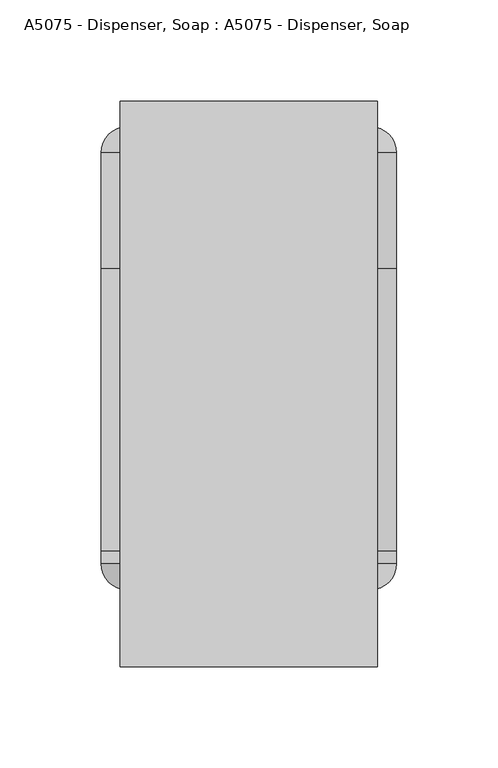
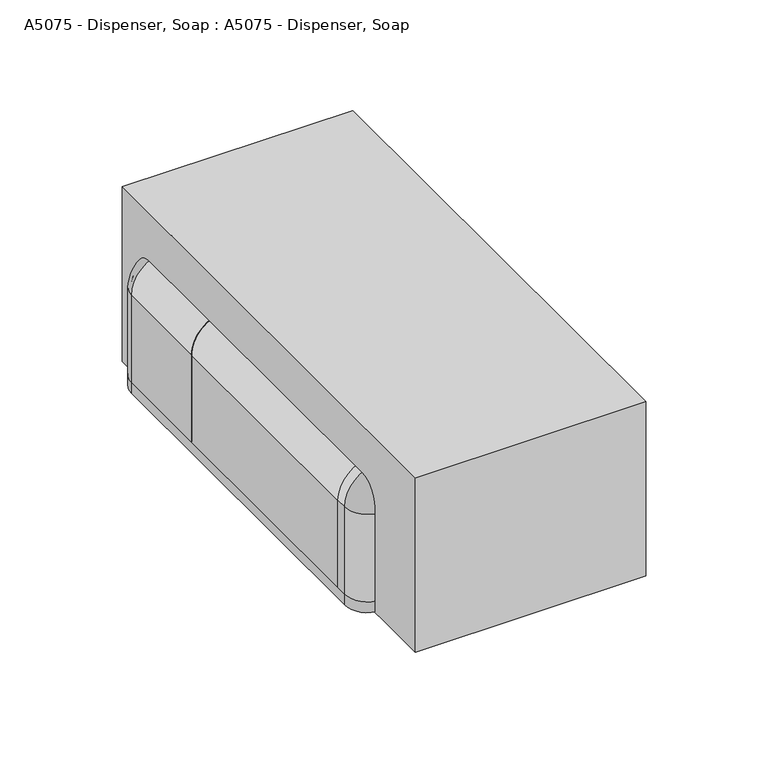
"""IFC4 building model written with IfcOpenShell, lengths in millimetres: proxy geometry, A5075 - Dispenser, Soap : A5075 - Dispenser, Soap."""

import ifcopenshell
import ifcopenshell.guid

model = None  # the IFC model being written
_history = None  # IfcOwnerHistory: only IFC2X3 demands one
_inside = {}  # id of a spatial element -> (the spatial element, [elements in it])
_under = {}  # id of a project, library or spatial element -> (it, [spatial elements below it])
_declared = {}  # id of a project -> (the project, [libraries it declares])
_typed = {}  # id of a type object -> (the type object, [elements of that type])
_made_of = {}  # id of a material, layer set ... -> (it, [elements and type objects made of it])


def new_model(schema):
    """Start an empty IFC model of exactly this schema.

    Asked for "IFC4X3", IfcOpenShell would pick the latest addendum, in which some entities
    have other attributes; the version numbers below select the first issue.
    IFC2X3 requires an IfcOwnerHistory on every rooted entity: one is made here for all.
    """
    global model, _history
    if schema == "IFC4X3":
        model = ifcopenshell.file(schema_version=(4, 3, 0, 0))
    else:
        model = ifcopenshell.file(schema=schema)
    _inside.clear()
    _under.clear()
    _declared.clear()
    _typed.clear()
    _made_of.clear()
    _history = None
    if model.schema == "IFC2X3":
        org = make("IfcOrganization", Name="unknown")
        user = make(
            "IfcPersonAndOrganization",
            ThePerson=make("IfcPerson", FamilyName="unknown"),
            TheOrganization=org,
        )
        app = make(
            "IfcApplication",
            ApplicationDeveloper=org,
            Version="unknown",
            ApplicationFullName="unknown",
            ApplicationIdentifier="unknown",
        )
        _history = make(
            "IfcOwnerHistory",
            OwningUser=user,
            OwningApplication=app,
            ChangeAction="ADDED",
            CreationDate=0,
        )
    return model


def make(cls, **values):
    """One entity of the class cls with the attributes given. An attribute that is None is left unset."""
    return model.create_entity(
        cls, **{name: value for name, value in values.items() if value is not None}
    )


def rooted(cls, **values):
    """An entity with a GlobalId (a new one), such as an element, a storey or a relation."""
    return make(cls, GlobalId=ifcopenshell.guid.new(), OwnerHistory=_history, **values)


def si_unit(unit_type, name, prefix=None):
    """IfcSIUnit, for example si_unit("LENGTHUNIT", "METRE", prefix="MILLI")."""
    return make("IfcSIUnit", UnitType=unit_type, Prefix=prefix, Name=name)


def assignment(units):
    """IfcUnitAssignment: the units of a project."""
    return None if units is None else make("IfcUnitAssignment", Units=units)


def point(xyz):
    """IfcCartesianPoint."""
    return None if xyz is None else make("IfcCartesianPoint", Coordinates=xyz)


def direction(xyz):
    """IfcDirection."""
    return None if xyz is None else make("IfcDirection", DirectionRatios=xyz)


def frame(location, z_axis=None, x_axis=None):
    """IfcAxis2Placement3D, a coordinate frame: its origin and axes. An axis left out is left unset."""
    return make(
        "IfcAxis2Placement3D",
        Location=point(location),
        Axis=direction(z_axis),
        RefDirection=direction(x_axis),
    )


def frame_2d(location, x_axis=None):
    """IfcAxis2Placement2D, a coordinate frame in the plane: its origin and x axis."""
    return make(
        "IfcAxis2Placement2D", Location=point(location), RefDirection=direction(x_axis)
    )


def origin():
    """The frame at (0, 0, 0) with its axes left unset."""
    return frame((0.0, 0.0, 0.0))


def origin_with_axes():
    """The frame at (0, 0, 0) with the z axis (0, 0, 1) and the x axis (1, 0, 0) written out."""
    return frame((0.0, 0.0, 0.0), z_axis=(0.0, 0.0, 1.0), x_axis=(1.0, 0.0, 0.0))


def place(relative_to, where):
    """IfcLocalPlacement: puts the frame where relative to a parent placement (None: the world)."""
    return make(
        "IfcLocalPlacement", PlacementRelTo=relative_to, RelativePlacement=where
    )


def context(
    kind, dimensions, precision=None, world=None, true_north=None, identifier=None
):
    """IfcGeometricRepresentationContext, for example the 3D "Model" context."""
    return make(
        "IfcGeometricRepresentationContext",
        ContextIdentifier=identifier,
        ContextType=kind,
        CoordinateSpaceDimension=dimensions,
        Precision=precision,
        WorldCoordinateSystem=world,
        TrueNorth=true_north,
    )


def project(units=None, contexts=None):
    """IfcProject with its units and contexts."""
    return rooted(
        "IfcProject",
        Name="project",
        RepresentationContexts=contexts,
        UnitsInContext=assignment(units),
    )


def spatial(cls, under=None, at=None, **own):
    """A site, building, storey or space (cls), placed at a placement, below another one or the project."""
    s = rooted(cls, ObjectPlacement=at, **own)
    if under is not None:
        _under.setdefault(under.id(), (under, []))[1].append(s)
    return s


def polyline(points):
    """IfcPolyline through the points."""
    return make("IfcPolyline", Points=[point(p) for p in points])


def circle_curve(where, radius):
    """IfcCircle in the frame where."""
    return make("IfcCircle", Position=where, Radius=radius)


def ellipse_curve(where, semi_axis1, semi_axis2):
    """IfcEllipse in the frame where."""
    return make(
        "IfcEllipse", Position=where, SemiAxis1=semi_axis1, SemiAxis2=semi_axis2
    )


def trimmed(basis, trim1, trim2, sense, master):
    """IfcTrimmedCurve: the piece of a basis curve between two trims."""
    return make(
        "IfcTrimmedCurve",
        BasisCurve=basis,
        Trim1=trim1,
        Trim2=trim2,
        SenseAgreement=sense,
        MasterRepresentation=master,
    )


def segment(curve, same_sense, transition):
    """IfcCompositeCurveSegment."""
    return make(
        "IfcCompositeCurveSegment",
        Transition=transition,
        SameSense=same_sense,
        ParentCurve=curve,
    )


def composite_curve(segments, self_intersect=None):
    """IfcCompositeCurve: segments joined end to end."""
    return make("IfcCompositeCurve", Segments=segments, SelfIntersect=self_intersect)


def outline(outer, holes=None, kind="AREA"):
    """IfcArbitraryClosedProfileDef: a profile drawn as a closed curve; with holes, ...WithVoids."""
    if holes is None:
        return make("IfcArbitraryClosedProfileDef", ProfileType=kind, OuterCurve=outer)
    return make(
        "IfcArbitraryProfileDefWithVoids",
        ProfileType=kind,
        OuterCurve=outer,
        InnerCurves=holes,
    )


def extrude(swept, where, along, depth):
    """IfcExtrudedAreaSolid: the profile swept, set in the frame where, extruded along a direction by depth."""
    return make(
        "IfcExtrudedAreaSolid",
        SweptArea=swept,
        Position=where,
        ExtrudedDirection=direction(along),
        Depth=depth,
    )


def shape(context_of_items, identifier, shape_type, items):
    """IfcShapeRepresentation: the items that make up one representation, for example the "Body"."""
    return make(
        "IfcShapeRepresentation",
        ContextOfItems=context_of_items,
        RepresentationIdentifier=identifier,
        RepresentationType=shape_type,
        Items=items,
    )


def source(mapping_origin, context_of_items, identifier, shape_type, items):
    """IfcRepresentationMap: a shape defined once, which mapped items show again and again."""
    return make(
        "IfcRepresentationMap",
        MappingOrigin=mapping_origin,
        MappedRepresentation=shape(context_of_items, identifier, shape_type, items),
    )


def transform(
    local_origin,
    x_axis=None,
    y_axis=None,
    z_axis=None,
    scale=None,
    scale2=None,
    scale3=None,
    uniform=True,
):
    """IfcCartesianTransformationOperator3D, or its non-uniform kind. x_axis, y_axis, z_axis: its Axis1, 2, 3."""
    if uniform:
        return make(
            "IfcCartesianTransformationOperator3D",
            Axis1=direction(x_axis),
            Axis2=direction(y_axis),
            LocalOrigin=point(local_origin),
            Scale=scale,
            Axis3=direction(z_axis),
        )
    return make(
        "IfcCartesianTransformationOperator3DnonUniform",
        Axis1=direction(x_axis),
        Axis2=direction(y_axis),
        LocalOrigin=point(local_origin),
        Scale=scale,
        Axis3=direction(z_axis),
        Scale2=scale2,
        Scale3=scale3,
    )


def mapped(mapping_source, mapping_target):
    """IfcMappedItem: shows the shape of a source again, moved by a transform."""
    return make(
        "IfcMappedItem", MappingSource=mapping_source, MappingTarget=mapping_target
    )


def made_of(thing, what):
    """Note that an element or type object is made of a material, layer set ...; save() writes the relation."""
    if what is not None:
        _made_of.setdefault(what.id(), (what, []))[1].append(thing)
    return thing


def element(
    cls,
    number,
    at=None,
    inside=None,
    cuts=None,
    type_object=None,
    material=None,
    context=None,
    identifier="Body",
    shape_type=None,
    held_by="IfcProductDefinitionShape",
    body=None,
    shapes=None,
    **own,
):
    """One element of the class cls, such as IfcWall. Its Tag is "e" and its number.

    at: its placement. inside: the storey or other place that contains it. cuts: it is an
    opening in that element (IfcRelVoidsElement). A single representation is given by context,
    identifier, shape_type and body (its items); several are given by shapes. held_by: the class
    of the entity that holds the representations. save() writes the other relations.
    """
    e = rooted(cls, Tag="e%d" % number, ObjectPlacement=at, **own)
    if body is not None:
        shapes = [shape(context, identifier, shape_type, body)]
    if shapes is not None:
        e.Representation = make(held_by, Representations=shapes)
    if inside is not None:
        _inside.setdefault(inside.id(), (inside, []))[1].append(e)
    if cuts is not None:
        rooted(
            "IfcRelVoidsElement", RelatingBuildingElement=cuts, RelatedOpeningElement=e
        )
    if type_object is not None:
        _typed.setdefault(type_object.id(), (type_object, []))[1].append(e)
    return made_of(e, material)


def aggregate(whole, parts):
    """IfcRelAggregates: a whole, such as a stair, and the parts it consists of."""
    return rooted("IfcRelAggregates", RelatingObject=whole, RelatedObjects=parts)


def save(model, path):
    """Write the relations noted so far, then the file.

    IfcRelAggregates (storeys below a building ...), IfcRelContainedInSpatialStructure (elements
    in a storey), IfcRelDefinesByType, IfcRelAssociatesMaterial and IfcRelDeclares: one each for
    every whole, place, type object, material and project.
    """
    for whole, parts in _under.values():
        aggregate(whole, parts)
    for where, things in _inside.values():
        rooted(
            "IfcRelContainedInSpatialStructure",
            RelatedElements=things,
            RelatingStructure=where,
        )
    for kind, things in _typed.values():
        rooted("IfcRelDefinesByType", RelatedObjects=things, RelatingType=kind)
    for what, things in _made_of.values():
        rooted("IfcRelAssociatesMaterial", RelatedObjects=things, RelatingMaterial=what)
    for by, libraries in _declared.values():
        rooted("IfcRelDeclares", RelatingContext=by, RelatedDefinitions=libraries)
    model.write(path)


def plane_surface(at):
    """IfcPlane: the flat surface through the origin of the frame at, square to its z axis."""
    return make("IfcPlane", Position=at)


def cylinder_surface(at, radius):
    """IfcCylindricalSurface: all points at the distance radius from the z axis of the frame at."""
    return make("IfcCylindricalSurface", Position=at, Radius=radius)


def revolved_surface(curve, axis_point, axis_direction):
    """IfcSurfaceOfRevolution: the curve turned about the line through axis_point along axis_direction."""
    return make(
        "IfcSurfaceOfRevolution",
        SweptCurve=make("IfcArbitraryOpenProfileDef", ProfileType="CURVE", Curve=curve),
        AxisPosition=make("IfcAxis1Placement", Location=point(axis_point), Axis=direction(axis_direction)),
    )


def advanced_brep(points, edges, surfaces, faces):
    """IfcAdvancedBrep: a solid bounded by faces that lie on surfaces and meet in shared edges.

    An edge is (start, end): straight between two places in points (the first is 0);
    or (start, end, curve); or (start, end, curve, False) where it runs against its curve.
    A face is (place in surfaces, loops), or (place, loops, False) where it looks against
    its surface's normal. A loop lists edges by number (the first is 1), with a minus sign
    where the edge is run from its end to its start. The first loop is the outer one.
    """
    corners = [point(p) for p in points]
    vertices = [make("IfcVertexPoint", VertexGeometry=c) for c in corners]
    made = []
    for start, end, *more in edges:
        made.append(
            make(
                "IfcEdgeCurve",
                EdgeStart=vertices[start],
                EdgeEnd=vertices[end],
                EdgeGeometry=more[0] if more else make("IfcPolyline", Points=[corners[start], corners[end]]),
                SameSense=more[1] if len(more) > 1 else True,
            )
        )
    hull = []
    for where, loops, *sense in faces:
        bounds = []
        for j, loop in enumerate(loops):
            ring = [make("IfcOrientedEdge", EdgeElement=made[abs(k) - 1], Orientation=k > 0) for k in loop]
            bounds.append(
                make(
                    "IfcFaceOuterBound" if j == 0 else "IfcFaceBound",
                    Bound=make("IfcEdgeLoop", EdgeList=ring),
                    Orientation=True,
                )
            )
        hull.append(make("IfcAdvancedFace", Bounds=bounds, FaceSurface=surfaces[where], SameSense=sense[0] if sense else True))
    return make("IfcAdvancedBrep", Outer=make("IfcClosedShell", CfsFaces=hull))


def a5075_dispenser_soap_a5075_dispenser_soap_cc7686cf(model_context):
    return source(origin(), model_context, "Body", "SolidModel", [
        advanced_brep(
        [(-73.025, -25.4, 6.35), (-60.325, -12.7, 6.35), (-60.325, -14.2875, 6.35), (-71.4375, -25.4, 6.35), (-71.4375, -82.55, 6.35), (-73.025, -82.55, 6.35), (-73.025, -82.55, 57.15), (-73.025, -25.4, 57.15), (-71.4375, -82.55, 57.15), (-53.975, -82.55, 74.6125), (53.975, -82.55, 74.6125), (71.4375, -82.55, 57.15), (71.4375, -82.55, 6.35), (73.025, -82.55, 6.35), (73.025, -82.55, 57.15), (53.975, -82.55, 76.2), (-53.975, -82.55, 76.2), (-71.4375, -25.4, 57.15), (-60.325, -14.2875, 57.15), (-60.325, -12.7, 57.15), (-53.975, -25.4, 76.2), (-53.975, -25.4, 74.6125), (-53.975, -14.2875, 63.5), (-53.975, -12.7, 63.5), (53.975, -25.4, 76.2), (53.975, -25.4, 74.6125), (53.975, -14.2875, 63.5), (53.975, -12.7, 63.5), (73.025, -25.4, 57.15), (71.4375, -25.4, 57.15), (60.325, -14.2875, 57.15), (60.325, -12.7, 57.15), (73.025, -25.4, 6.35), (71.4375, -25.4, 6.35), (60.325, -14.2875, 6.35), (60.325, -12.7, 6.35)],
        [
            (0, 1, circle_curve(frame((-60.325, -25.4, 6.35), z_axis=(0.0, 0.0, -1.0), x_axis=(1.0, 0.0, 0.0)), 12.7)),
            (1, 2),
            (2, 3, circle_curve(frame((-60.325, -25.4, 6.35), z_axis=(0.0, 0.0, 1.0), x_axis=(1.0, 0.0, 0.0)), 11.1125)),
            (3, 4),
            (4, 5),
            (5, 0),
            (5, 6),
            (6, 7),
            (7, 0),
            (4, 8),
            (8, 9, circle_curve(frame((-53.975, -82.55, 57.15), z_axis=(0.0, 1.0, 0.0), x_axis=(-1.0, 0.0, 0.0)), 17.4625)),
            (9, 10),
            (10, 11, circle_curve(frame((53.975, -82.55, 57.15), z_axis=(0.0, 1.0, 0.0), x_axis=(0.0, 0.0, 1.0)), 17.4625)),
            (11, 12),
            (12, 13),
            (13, 14),
            (14, 15, circle_curve(frame((53.975, -82.55, 57.15), z_axis=(0.0, -1.0, 0.0), x_axis=(0.0, 0.0, 1.0)), 19.05)),
            (15, 16),
            (16, 6, circle_curve(frame((-53.975, -82.55, 57.15), z_axis=(0.0, -1.0, 0.0), x_axis=(-1.0, 0.0, 0.0)), 19.05)),
            (3, 17),
            (17, 8),
            (2, 18),
            (18, 17, circle_curve(frame((-60.325, -25.4, 57.15), z_axis=(0.0, 0.0, 1.0), x_axis=(1.0, 0.0, 0.0)), 11.1125)),
            (1, 19),
            (19, 18),
            (7, 19, circle_curve(frame((-60.325, -25.4, 57.15), z_axis=(0.0, 0.0, -1.0), x_axis=(1.0, 0.0, 0.0)), 12.7)),
            (16, 20),
            (20, 7, circle_curve(frame((-53.975, -25.4, 57.15), z_axis=(0.0, -1.0, 0.0), x_axis=(-1.0, 0.0, 0.0)), 19.05)),
            (21, 9),
            (17, 21, circle_curve(frame((-53.975, -25.4, 57.15), z_axis=(0.0, 1.0, 0.0), x_axis=(-1.0, 0.0, 0.0)), 17.4625)),
            (22, 21, circle_curve(frame((-53.975, -25.4, 63.5), z_axis=(1.0, 0.0, 0.0), x_axis=(0.0, 0.0, -1.0)), 11.1125)),
            (18, 22, circle_curve(frame((-53.975, -14.2875, 57.15), z_axis=(0.0, 1.0, 0.0), x_axis=(-1.0, 0.0, 0.0)), 6.35)),
            (23, 22),
            (19, 23, circle_curve(frame((-53.975, -12.7, 57.15), z_axis=(0.0, 1.0, 0.0), x_axis=(-1.0, 0.0, 0.0)), 6.35)),
            (20, 23, circle_curve(frame((-53.975, -25.4, 63.5), z_axis=(-1.0, 0.0, 0.0), x_axis=(0.0, 0.0, -1.0)), 12.7)),
            (15, 24),
            (24, 20),
            (21, 25),
            (25, 10),
            (22, 26),
            (26, 25, circle_curve(frame((53.975, -25.4, 63.5), z_axis=(1.0, 0.0, 0.0), x_axis=(0.0, 0.0, -1.0)), 11.1125)),
            (23, 27),
            (27, 26),
            (24, 27, circle_curve(frame((53.975, -25.4, 63.5), z_axis=(-1.0, 0.0, 0.0), x_axis=(0.0, 0.0, -1.0)), 12.7)),
            (14, 28),
            (28, 24, circle_curve(frame((53.975, -25.4, 57.15), z_axis=(0.0, -1.0, 0.0), x_axis=(0.0, 0.0, 1.0)), 19.05)),
            (29, 11),
            (25, 29, circle_curve(frame((53.975, -25.4, 57.15), z_axis=(0.0, 1.0, 0.0), x_axis=(0.0, 0.0, 1.0)), 17.4625)),
            (30, 29, circle_curve(frame((60.325, -25.4, 57.15), z_axis=(0.0, 0.0, -1.0), x_axis=(-1.0, 0.0, 0.0)), 11.1125)),
            (26, 30, circle_curve(frame((53.975, -14.2875, 57.15), z_axis=(0.0, 1.0, 0.0), x_axis=(0.0, 0.0, 1.0)), 6.35)),
            (31, 30),
            (27, 31, circle_curve(frame((53.975, -12.7, 57.15), z_axis=(0.0, 1.0, 0.0), x_axis=(0.0, 0.0, 1.0)), 6.35)),
            (28, 31, circle_curve(frame((60.325, -25.4, 57.15), z_axis=(0.0, 0.0, 1.0), x_axis=(-1.0, 0.0, 0.0)), 12.7)),
            (32, 13),
            (12, 33),
            (33, 34, circle_curve(frame((60.325, -25.4, 6.35), z_axis=(0.0, 0.0, 1.0), x_axis=(-1.0, 0.0, 0.0)), 11.1125)),
            (34, 35),
            (35, 32, circle_curve(frame((60.325, -25.4, 6.35), z_axis=(0.0, 0.0, -1.0), x_axis=(-1.0, 0.0, 0.0)), 12.7)),
            (32, 28),
            (29, 33),
            (30, 34),
            (31, 35),
        ],
        [
            plane_surface(frame((-73.025, -12.7, 6.35), z_axis=(0.0, 0.0, -1.0), x_axis=(0.0, -1.0, 0.0))),
            plane_surface(frame((-73.025, -25.4, 6.35), z_axis=(-1.0, 0.0, 0.0), x_axis=(0.0, 0.0, 1.0))),
            plane_surface(frame((-73.025, -82.55, 6.35), z_axis=(0.0, -1.0, 0.0), x_axis=(0.0, 0.0, 1.0))),
            plane_surface(frame((-71.4375, -82.55, 6.35), z_axis=(1.0, 0.0, 0.0), x_axis=(0.0, 0.0, 1.0))),
            revolved_surface(polyline([(-49.212500000000006, -25.4, 57.15), (-49.212500000000006, -25.4, 6.35)]), (-60.325, -25.4, 6.35), (0.0, 0.0, 1.0)),
            plane_surface(frame((-60.325, -14.2875, 6.35), z_axis=(1.0, 0.0, 0.0), x_axis=(0.0, 0.0, 1.0))),
            cylinder_surface(frame((-60.325, -25.4, 6.35), z_axis=(0.0, 0.0, -1.0), x_axis=(1.0, 0.0, 0.0)), 12.7),
            cylinder_surface(frame((-53.975, -12.7, 57.15), z_axis=(0.0, -1.0, 0.0), x_axis=(-1.0, 0.0, 0.0)), 19.05),
            revolved_surface(polyline([(-71.4375, -82.55, 57.15), (-71.4375, -25.4, 57.15)]), (-53.975, -12.7, 57.15), (0.0, -1.0, 0.0)),
            revolved_surface(trimmed(ellipse_curve(frame((-60.325, -25.4, 57.15), z_axis=(0.0, 0.0, -1.0), x_axis=(1.0, 0.0, 0.0)), 11.1125, 11.1125), [point((-71.4375, -25.4, 57.15))], [point((-60.325, -14.2875, 57.15))], True, "CARTESIAN"), (-53.975, -12.7, 57.15), (0.0, -1.0, 0.0)),
            revolved_surface(polyline([(-60.325, -14.2875, 57.15), (-60.325, -12.7, 57.15)]), (-53.975, -12.7, 57.15), (0.0, -1.0, 0.0)),
            revolved_surface(trimmed(ellipse_curve(frame((-60.325, -25.4, 57.15), z_axis=(0.0, 0.0, 1.0), x_axis=(1.0, 0.0, 0.0)), 12.7, 12.7), [point((-60.325, -12.7, 57.15))], [point((-73.025, -25.4, 57.15))], True, "CARTESIAN"), (-53.975, -12.7, 57.15), (0.0, -1.0, 0.0)),
            plane_surface(frame((-53.975, -25.4, 76.2), z_axis=(0.0, 0.0, 1.0), x_axis=(1.0, 0.0, 0.0))),
            plane_surface(frame((-53.975, -82.55, 74.6125), z_axis=(0.0, 0.0, -1.0), x_axis=(1.0, 0.0, 0.0))),
            revolved_surface(polyline([(53.975, -25.4, 52.3875), (-53.975, -25.4, 52.3875)]), (-53.975, -25.4, 63.5), (1.0, 0.0, 0.0)),
            plane_surface(frame((-53.975, -14.2875, 63.5), z_axis=(0.0, 0.0, -1.0), x_axis=(1.0, 0.0, 0.0))),
            cylinder_surface(frame((-53.975, -25.4, 63.5), z_axis=(-1.0, 0.0, 0.0), x_axis=(0.0, 0.0, -1.0)), 12.7),
            cylinder_surface(frame((53.975, -12.7, 57.15), z_axis=(0.0, -1.0, 0.0), x_axis=(0.0, 0.0, 1.0)), 19.05),
            revolved_surface(polyline([(53.975, -82.55, 74.6125), (53.975, -25.4, 74.6125)]), (53.975, -12.7, 57.15), (0.0, -1.0, 0.0)),
            revolved_surface(trimmed(ellipse_curve(frame((53.975, -25.4, 63.5), z_axis=(-1.0, 0.0, 0.0), x_axis=(0.0, 0.0, -1.0)), 11.1125, 11.1125), [point((53.975, -25.4, 74.6125))], [point((53.975, -14.2875, 63.5))], True, "CARTESIAN"), (53.975, -12.7, 57.15), (0.0, -1.0, 0.0)),
            revolved_surface(polyline([(53.975, -14.2875, 63.5), (53.975, -12.7, 63.5)]), (53.975, -12.7, 57.15), (0.0, -1.0, 0.0)),
            revolved_surface(trimmed(ellipse_curve(frame((53.975, -25.4, 63.5), z_axis=(1.0, 0.0, 0.0), x_axis=(0.0, 0.0, -1.0)), 12.7, 12.7), [point((53.975, -12.7, 63.5))], [point((53.975, -25.4, 76.2))], True, "CARTESIAN"), (53.975, -12.7, 57.15), (0.0, -1.0, 0.0)),
            plane_surface(frame((73.025, -12.7, 6.35), z_axis=(0.0, 0.0, -1.0), x_axis=(0.0, -1.0, 0.0))),
            plane_surface(frame((73.025, -25.4, 57.15), z_axis=(1.0, 0.0, 0.0), x_axis=(0.0, 0.0, -1.0))),
            plane_surface(frame((71.4375, -82.55, 57.15), z_axis=(-1.0, 0.0, 0.0), x_axis=(0.0, 0.0, -1.0))),
            revolved_surface(polyline([(49.212500000000006, -25.4, 6.350000000000001), (49.212500000000006, -25.4, 57.15)]), (60.325, -25.4, 57.15), (0.0, 0.0, -1.0)),
            plane_surface(frame((60.325, -14.2875, 57.15), z_axis=(-1.0, 0.0, 0.0), x_axis=(0.0, 0.0, -1.0))),
            cylinder_surface(frame((60.325, -25.4, 57.15), z_axis=(0.0, 0.0, 1.0), x_axis=(-1.0, 0.0, 0.0)), 12.7),
        ],
        [
            (0, [[1, 2, 3, 4, 5, 6]]),
            (1, [[7, 8, 9, -6]]),
            (2, [[10, 11, 12, 13, 14, 15, 16, 17, 18, 19, -7, -5]]),
            (3, [[20, 21, -10, -4]]),
            (4, [[22, 23, -20, -3]]),
            (5, [[24, 25, -22, -2]]),
            (6, [[-9, 26, -24, -1]]),
            (7, [[27, 28, -8, -19]]),
            (8, [[29, -11, -21, 30]]),
            (9, [[31, -30, -23, 32]]),
            (10, [[33, -32, -25, 34]]),
            (11, [[35, -34, -26, -28]]),
            (12, [[-18, 36, 37, -27]]),
            (13, [[38, 39, -12, -29]]),
            (14, [[40, 41, -38, -31]]),
            (15, [[42, 43, -40, -33]]),
            (16, [[-37, 44, -42, -35]]),
            (17, [[45, 46, -36, -17]]),
            (18, [[47, -13, -39, 48]]),
            (19, [[49, -48, -41, 50]]),
            (20, [[51, -50, -43, 52]]),
            (21, [[53, -52, -44, -46]]),
            (22, [[54, -15, 55, 56, 57, 58]]),
            (23, [[-16, -54, 59, -45]]),
            (24, [[60, -55, -14, -47]]),
            (25, [[61, -56, -60, -49]]),
            (26, [[62, -57, -61, -51]]),
            (27, [[-59, -58, -62, -53]]),
        ],
    ),
        advanced_brep(
        [(-73.025, -228.6, 6.35), (-73.025, -222.25, 6.35), (-71.4375, -222.25, 6.35), (-71.4375, -228.6, 6.35), (-60.325, -239.7125, 6.35), (-60.325, -241.3, 6.35), (-60.325, -241.3, 57.15), (-73.025, -228.6, 57.15), (-60.325, -239.7125, 57.15), (-71.4375, -228.6, 57.15), (-71.4375, -222.25, 57.15), (-73.025, -222.25, 57.15), (-53.975, -222.25, 76.2), (53.975, -222.25, 76.2), (73.025, -222.25, 57.15), (73.025, -222.25, 6.35), (71.4375, -222.25, 6.35), (71.4375, -222.25, 57.15), (53.975, -222.25, 74.6125), (-53.975, -222.25, 74.6125), (-53.975, -241.3, 63.5), (-53.975, -228.6, 76.2), (-53.975, -239.7125, 63.5), (-53.975, -228.6, 74.6125), (53.975, -241.3, 63.5), (53.975, -228.6, 76.2), (53.975, -239.7125, 63.5), (53.975, -228.6, 74.6125), (60.325, -241.3, 57.15), (73.025, -228.6, 57.15), (60.325, -239.7125, 57.15), (71.4375, -228.6, 57.15), (73.025, -228.6, 6.35), (60.325, -241.3, 6.35), (60.325, -239.7125, 6.35), (71.4375, -228.6, 6.35)],
        [
            (0, 1),
            (1, 2),
            (2, 3),
            (3, 4, circle_curve(frame((-60.325, -228.6, 6.35), z_axis=(0.0, 0.0, 1.0), x_axis=(1.0, 0.0, 0.0)), 11.1125)),
            (4, 5),
            (5, 0, circle_curve(frame((-60.325, -228.6, 6.35), z_axis=(0.0, 0.0, -1.0), x_axis=(1.0, 0.0, 0.0)), 12.7)),
            (5, 6),
            (6, 7, circle_curve(frame((-60.325, -228.6, 57.15), z_axis=(0.0, 0.0, -1.0), x_axis=(1.0, 0.0, 0.0)), 12.7)),
            (7, 0),
            (4, 8),
            (8, 6),
            (3, 9),
            (9, 8, circle_curve(frame((-60.325, -228.6, 57.15), z_axis=(0.0, 0.0, 1.0), x_axis=(1.0, 0.0, 0.0)), 11.1125)),
            (2, 10),
            (10, 9),
            (1, 11),
            (11, 12, circle_curve(frame((-53.975, -222.25, 57.15), z_axis=(0.0, 1.0, 0.0), x_axis=(-1.0, 0.0, 0.0)), 19.05)),
            (12, 13),
            (13, 14, circle_curve(frame((53.975, -222.25, 57.15), z_axis=(0.0, 1.0, 0.0), x_axis=(0.0, 0.0, 1.0)), 19.05)),
            (14, 15),
            (15, 16),
            (16, 17),
            (17, 18, circle_curve(frame((53.975, -222.25, 57.15), z_axis=(0.0, -1.0, 0.0), x_axis=(0.0, 0.0, 1.0)), 17.4625)),
            (18, 19),
            (19, 10, circle_curve(frame((-53.975, -222.25, 57.15), z_axis=(0.0, -1.0, 0.0), x_axis=(-1.0, 0.0, 0.0)), 17.4625)),
            (7, 11),
            (20, 21, circle_curve(frame((-53.975, -228.6, 63.5), z_axis=(-1.0, 0.0, 0.0), x_axis=(0.0, 0.0, -1.0)), 12.7)),
            (21, 7, circle_curve(frame((-53.975, -228.6, 57.15), z_axis=(0.0, -1.0, 0.0), x_axis=(-1.0, 0.0, 0.0)), 19.05)),
            (6, 20, circle_curve(frame((-53.975, -241.3, 57.15), z_axis=(0.0, 1.0, 0.0), x_axis=(-1.0, 0.0, 0.0)), 6.35)),
            (22, 20),
            (8, 22, circle_curve(frame((-53.975, -239.7125, 57.15), z_axis=(0.0, 1.0, 0.0), x_axis=(-1.0, 0.0, 0.0)), 6.35)),
            (23, 22, circle_curve(frame((-53.975, -228.6, 63.5), z_axis=(1.0, 0.0, 0.0), x_axis=(0.0, 0.0, -1.0)), 11.1125)),
            (9, 23, circle_curve(frame((-53.975, -228.6, 57.15), z_axis=(0.0, 1.0, 0.0), x_axis=(-1.0, 0.0, 0.0)), 17.4625)),
            (19, 23),
            (21, 12),
            (20, 24),
            (24, 25, circle_curve(frame((53.975, -228.6, 63.5), z_axis=(-1.0, 0.0, 0.0), x_axis=(0.0, 0.0, -1.0)), 12.7)),
            (25, 21),
            (22, 26),
            (26, 24),
            (23, 27),
            (27, 26, circle_curve(frame((53.975, -228.6, 63.5), z_axis=(1.0, 0.0, 0.0), x_axis=(0.0, 0.0, -1.0)), 11.1125)),
            (18, 27),
            (25, 13),
            (28, 29, circle_curve(frame((60.325, -228.6, 57.15), z_axis=(0.0, 0.0, 1.0), x_axis=(-1.0, 0.0, 0.0)), 12.7)),
            (29, 25, circle_curve(frame((53.975, -228.6, 57.15), z_axis=(0.0, -1.0, 0.0), x_axis=(0.0, 0.0, 1.0)), 19.05)),
            (24, 28, circle_curve(frame((53.975, -241.3, 57.15), z_axis=(0.0, 1.0, 0.0), x_axis=(0.0, 0.0, 1.0)), 6.35)),
            (30, 28),
            (26, 30, circle_curve(frame((53.975, -239.7125, 57.15), z_axis=(0.0, 1.0, 0.0), x_axis=(0.0, 0.0, 1.0)), 6.35)),
            (31, 30, circle_curve(frame((60.325, -228.6, 57.15), z_axis=(0.0, 0.0, -1.0), x_axis=(-1.0, 0.0, 0.0)), 11.1125)),
            (27, 31, circle_curve(frame((53.975, -228.6, 57.15), z_axis=(0.0, 1.0, 0.0), x_axis=(0.0, 0.0, 1.0)), 17.4625)),
            (17, 31),
            (29, 14),
            (32, 33, circle_curve(frame((60.325, -228.6, 6.35), z_axis=(0.0, 0.0, -1.0), x_axis=(-1.0, 0.0, 0.0)), 12.7)),
            (33, 34),
            (34, 35, circle_curve(frame((60.325, -228.6, 6.35), z_axis=(0.0, 0.0, 1.0), x_axis=(-1.0, 0.0, 0.0)), 11.1125)),
            (35, 16),
            (15, 32),
            (28, 33),
            (32, 29),
            (30, 34),
            (31, 35),
        ],
        [
            plane_surface(frame((-73.025, -241.3, 6.35), z_axis=(0.0, 0.0, -1.0), x_axis=(0.0, -1.0, 0.0))),
            cylinder_surface(frame((-60.325, -228.6, 6.35), z_axis=(0.0, 0.0, -1.0), x_axis=(1.0, 0.0, 0.0)), 12.7),
            plane_surface(frame((-60.325, -241.3, 6.35), z_axis=(1.0, 0.0, 0.0), x_axis=(0.0, 0.0, 1.0))),
            revolved_surface(polyline([(-49.212500000000006, -228.6, 57.15), (-49.212500000000006, -228.6, 6.35)]), (-60.325, -228.6, 6.35), (0.0, 0.0, 1.0)),
            plane_surface(frame((-71.4375, -228.6, 6.35), z_axis=(1.0, 0.0, 0.0), x_axis=(0.0, 0.0, 1.0))),
            plane_surface(frame((-71.4375, -222.25, 6.35), z_axis=(0.0, 1.0, 0.0), x_axis=(0.0, 0.0, 1.0))),
            plane_surface(frame((-73.025, -222.25, 6.35), z_axis=(-1.0, 0.0, 0.0), x_axis=(0.0, 0.0, 1.0))),
            revolved_surface(trimmed(ellipse_curve(frame((-60.325, -228.6, 57.15), z_axis=(0.0, 0.0, 1.0), x_axis=(1.0, 0.0, 0.0)), 12.7, 12.7), [point((-73.025, -228.6, 57.15))], [point((-60.325, -241.3, 57.15))], True, "CARTESIAN"), (-53.975, -241.3, 57.15), (0.0, -1.0, 0.0)),
            revolved_surface(polyline([(-60.325, -241.3, 57.15), (-60.325, -239.7125, 57.15)]), (-53.975, -241.3, 57.15), (0.0, -1.0, 0.0)),
            revolved_surface(trimmed(ellipse_curve(frame((-60.325, -228.6, 57.15), z_axis=(0.0, 0.0, -1.0), x_axis=(1.0, 0.0, 0.0)), 11.1125, 11.1125), [point((-60.325, -239.7125, 57.15))], [point((-71.4375, -228.6, 57.15))], True, "CARTESIAN"), (-53.975, -241.3, 57.15), (0.0, -1.0, 0.0)),
            revolved_surface(polyline([(-71.4375, -228.6, 57.15), (-71.4375, -222.25, 57.15)]), (-53.975, -241.3, 57.15), (0.0, -1.0, 0.0)),
            cylinder_surface(frame((-53.975, -241.3, 57.15), z_axis=(0.0, -1.0, 0.0), x_axis=(-1.0, 0.0, 0.0)), 19.05),
            cylinder_surface(frame((-53.975, -228.6, 63.5), z_axis=(-1.0, 0.0, 0.0), x_axis=(0.0, 0.0, -1.0)), 12.7),
            plane_surface(frame((-53.975, -241.3, 63.5), z_axis=(0.0, 0.0, -1.0), x_axis=(1.0, 0.0, 0.0))),
            revolved_surface(polyline([(53.975, -228.6, 52.3875), (-53.975, -228.6, 52.3875)]), (-53.975, -228.6, 63.5), (1.0, 0.0, 0.0)),
            plane_surface(frame((-53.975, -228.6, 74.6125), z_axis=(0.0, 0.0, -1.0), x_axis=(1.0, 0.0, 0.0))),
            plane_surface(frame((-53.975, -222.25, 76.2), z_axis=(0.0, 0.0, 1.0), x_axis=(1.0, 0.0, 0.0))),
            revolved_surface(trimmed(ellipse_curve(frame((53.975, -228.6, 63.5), z_axis=(1.0, 0.0, 0.0), x_axis=(0.0, 0.0, -1.0)), 12.7, 12.7), [point((53.975, -228.6, 76.2))], [point((53.975, -241.3, 63.5))], True, "CARTESIAN"), (53.975, -241.3, 57.15), (0.0, -1.0, 0.0)),
            revolved_surface(polyline([(53.975, -241.3, 63.5), (53.975, -239.7125, 63.5)]), (53.975, -241.3, 57.15), (0.0, -1.0, 0.0)),
            revolved_surface(trimmed(ellipse_curve(frame((53.975, -228.6, 63.5), z_axis=(-1.0, 0.0, 0.0), x_axis=(0.0, 0.0, -1.0)), 11.1125, 11.1125), [point((53.975, -239.7125, 63.5))], [point((53.975, -228.6, 74.6125))], True, "CARTESIAN"), (53.975, -241.3, 57.15), (0.0, -1.0, 0.0)),
            revolved_surface(polyline([(53.975, -228.6, 74.6125), (53.975, -222.25, 74.6125)]), (53.975, -241.3, 57.15), (0.0, -1.0, 0.0)),
            cylinder_surface(frame((53.975, -241.3, 57.15), z_axis=(0.0, -1.0, 0.0), x_axis=(0.0, 0.0, 1.0)), 19.05),
            plane_surface(frame((73.025, -241.3, 6.35), z_axis=(0.0, 0.0, -1.0), x_axis=(0.0, -1.0, 0.0))),
            cylinder_surface(frame((60.325, -228.6, 57.15), z_axis=(0.0, 0.0, 1.0), x_axis=(-1.0, 0.0, 0.0)), 12.7),
            plane_surface(frame((60.325, -241.3, 57.15), z_axis=(-1.0, 0.0, 0.0), x_axis=(0.0, 0.0, -1.0))),
            revolved_surface(polyline([(49.212500000000006, -228.6, 6.350000000000001), (49.212500000000006, -228.6, 57.15)]), (60.325, -228.6, 57.15), (0.0, 0.0, -1.0)),
            plane_surface(frame((71.4375, -228.6, 57.15), z_axis=(-1.0, 0.0, 0.0), x_axis=(0.0, 0.0, -1.0))),
            plane_surface(frame((73.025, -222.25, 57.15), z_axis=(1.0, 0.0, 0.0), x_axis=(0.0, 0.0, -1.0))),
        ],
        [
            (0, [[1, 2, 3, 4, 5, 6]]),
            (1, [[7, 8, 9, -6]]),
            (2, [[10, 11, -7, -5]]),
            (3, [[12, 13, -10, -4]]),
            (4, [[14, 15, -12, -3]]),
            (5, [[16, 17, 18, 19, 20, 21, 22, 23, 24, 25, -14, -2]]),
            (6, [[-9, 26, -16, -1]]),
            (7, [[27, 28, -8, 29]]),
            (8, [[30, -29, -11, 31]]),
            (9, [[32, -31, -13, 33]]),
            (10, [[34, -33, -15, -25]]),
            (11, [[35, -17, -26, -28]]),
            (12, [[36, 37, 38, -27]]),
            (13, [[39, 40, -36, -30]]),
            (14, [[41, 42, -39, -32]]),
            (15, [[-24, 43, -41, -34]]),
            (16, [[-38, 44, -18, -35]]),
            (17, [[45, 46, -37, 47]]),
            (18, [[48, -47, -40, 49]]),
            (19, [[50, -49, -42, 51]]),
            (20, [[52, -51, -43, -23]]),
            (21, [[53, -19, -44, -46]]),
            (22, [[54, 55, 56, 57, -21, 58]]),
            (23, [[59, -54, 60, -45]]),
            (24, [[61, -55, -59, -48]]),
            (25, [[62, -56, -61, -50]]),
            (26, [[-22, -57, -62, -52]]),
            (27, [[-60, -58, -20, -53]]),
        ],
    ),
        extrude(outline(composite_curve([segment(polyline([(57.15, -73.025), (6.35, -73.025), (6.35, -71.4375), (57.15, -71.4375)]), True, "CONTINUOUS"), segment(trimmed(circle_curve(frame_2d((57.15, -53.975)), 17.4625), [point((57.15, -71.4375))], [point((74.6125, -53.975))], True, "CARTESIAN"), True, "CONTINUOUS"), segment(polyline([(74.6125, -53.975), (74.6125, 53.975)]), True, "CONTINUOUS"), segment(trimmed(circle_curve(frame_2d((57.15, 53.975)), 17.4625), [point((74.6125, 53.975))], [point((57.15, 71.4375))], True, "CARTESIAN"), True, "CONTINUOUS"), segment(polyline([(57.15, 71.4375), (6.35, 71.4375), (6.35, 73.025), (57.15, 73.025)]), True, "CONTINUOUS"), segment(trimmed(circle_curve(frame_2d((57.15, 53.975)), 19.05), [point((57.15, 73.025))], [point((76.2, 53.975))], False, "CARTESIAN"), True, "CONTINUOUS"), segment(polyline([(76.2, 53.975), (76.2, -53.975)]), True, "CONTINUOUS"), segment(trimmed(circle_curve(frame_2d((57.15, -53.975)), 19.05), [point((76.2, -53.975))], [point((57.15, -73.025))], False, "CARTESIAN"), True, "CONTINUOUS")], self_intersect=False)), frame((0.0, -222.25, 0.0), z_axis=(0.0, 1.0, 0.0), x_axis=(0.0, 0.0, 1.0)), (0.0, 0.0, 1.0), 139.7),
        extrude(outline(composite_curve([segment(polyline([(74.6125, 53.975), (74.6125, -53.975)]), True, "CONTINUOUS"), segment(trimmed(circle_curve(frame_2d((57.15, -53.975)), 17.4625), [point((74.6125, -53.975))], [point((57.15, -71.4375))], False, "CARTESIAN"), True, "CONTINUOUS"), segment(polyline([(57.15, -71.4375), (6.35, -71.4375), (6.35, 71.4375), (57.15, 71.4375)]), True, "CONTINUOUS"), segment(trimmed(circle_curve(frame_2d((57.15, 53.975)), 17.4625), [point((57.15, 71.4375))], [point((74.6125, 53.975))], False, "CARTESIAN"), True, "CONTINUOUS")], self_intersect=False)), frame((0.0, -184.4030988, 0.0), z_axis=(0.0, 1.0, 0.0), x_axis=(0.0, 0.0, 1.0)), (0.0, 0.0, 1.0), 101.8530988),
        extrude(outline(composite_curve([segment(trimmed(circle_curve(frame_2d((47.625, 0.0)), 9.525), [point((47.625, -9.525))], [point((47.625, 9.525))], False, "CARTESIAN"), True, "CONTINUOUS"), segment(trimmed(circle_curve(frame_2d((47.625, 0.0)), 9.525), [point((47.625, 9.525))], [point((47.625, -9.525))], False, "CARTESIAN"), True, "CONTINUOUS")], self_intersect=False)), frame((0.0, -12.7, 0.0), z_axis=(0.0, 1.0, 0.0), x_axis=(0.0, 0.0, 1.0)), (0.0, 0.0, 1.0), 12.7),
        extrude(outline(composite_curve([segment(trimmed(circle_curve(frame_2d((-9.525, -41.275)), 9.525), [point((-9.525, -50.8))], [point((-9.525, -31.75))], False, "CARTESIAN"), True, "CONTINUOUS"), segment(polyline([(-9.525, -31.75), (9.525, -31.75)]), True, "CONTINUOUS"), segment(trimmed(circle_curve(frame_2d((9.525, -41.275)), 9.525), [point((9.525, -31.75))], [point((9.525, -50.8))], False, "CARTESIAN"), True, "CONTINUOUS"), segment(polyline([(9.525, -50.8), (-9.525, -50.8)]), True, "CONTINUOUS")], self_intersect=False)), frame((0.0, 0.0, 76.2), z_axis=(0.0, 0.0, 1.0), x_axis=(1.0, 0.0, 0.0)), (0.0, 0.0, 1.0), 12.7),
        extrude(outline(composite_curve([segment(polyline([(6.35, -60.325), (6.35, 60.325), (57.15, 60.325)]), True, "CONTINUOUS"), segment(trimmed(circle_curve(frame_2d((57.15, 53.975)), 6.35), [point((57.15, 60.325))], [point((63.5, 53.975))], False, "CARTESIAN"), True, "CONTINUOUS"), segment(polyline([(63.5, 53.975), (63.5, -53.975)]), True, "CONTINUOUS"), segment(trimmed(circle_curve(frame_2d((57.15, -53.975)), 6.35), [point((63.5, -53.975))], [point((57.15, -60.325))], False, "CARTESIAN"), True, "CONTINUOUS"), segment(polyline([(57.15, -60.325), (6.35, -60.325)]), True, "CONTINUOUS")], self_intersect=False)), frame((0.0, -14.2875, 0.0), z_axis=(0.0, 1.0, 0.0), x_axis=(0.0, 0.0, 1.0)), (0.0, 0.0, 1.0), 1.5875),
        extrude(outline(composite_curve([segment(trimmed(circle_curve(frame_2d((-60.325, -228.6)), 12.7), [point((-60.325, -241.3))], [point((-73.025, -228.6))], False, "CARTESIAN"), True, "CONTINUOUS"), segment(polyline([(-73.025, -228.6), (-73.025, -25.4)]), True, "CONTINUOUS"), segment(trimmed(circle_curve(frame_2d((-60.325, -25.4)), 12.7), [point((-73.025, -25.4))], [point((-60.325, -12.7))], False, "CARTESIAN"), True, "CONTINUOUS"), segment(polyline([(-60.325, -12.7), (60.325, -12.7)]), True, "CONTINUOUS"), segment(trimmed(circle_curve(frame_2d((60.325, -25.4)), 12.7), [point((60.325, -12.7))], [point((73.025, -25.4))], False, "CARTESIAN"), True, "CONTINUOUS"), segment(polyline([(73.025, -25.4), (73.025, -228.6)]), True, "CONTINUOUS"), segment(trimmed(circle_curve(frame_2d((60.325, -228.6)), 12.7), [point((73.025, -228.6))], [point((60.325, -241.3))], False, "CARTESIAN"), True, "CONTINUOUS"), segment(polyline([(60.325, -241.3), (-60.325, -241.3)]), True, "CONTINUOUS")], self_intersect=False)), origin_with_axes(), (0.0, 0.0, 1.0), 6.35),
        extrude(outline(polyline([(63.5, -279.4), (-63.5, -279.4), (-63.5, 0.0), (63.5, 0.0), (63.5, -279.4)])), origin_with_axes(), (0.0, 0.0, 1.0), 101.6),
        extrude(outline(composite_curve([segment(polyline([(6.35, -60.325), (6.35, 60.325), (57.15, 60.325)]), True, "CONTINUOUS"), segment(trimmed(circle_curve(frame_2d((57.15, 53.975)), 6.35), [point((57.15, 60.325))], [point((63.5, 53.975))], False, "CARTESIAN"), True, "CONTINUOUS"), segment(polyline([(63.5, 53.975), (63.5, -53.975)]), True, "CONTINUOUS"), segment(trimmed(circle_curve(frame_2d((57.15, -53.975)), 6.35), [point((63.5, -53.975))], [point((57.15, -60.325))], False, "CARTESIAN"), True, "CONTINUOUS"), segment(polyline([(57.15, -60.325), (6.35, -60.325)]), True, "CONTINUOUS")], self_intersect=False)), frame((0.0, -241.3, 0.0), z_axis=(0.0, 1.0, 0.0), x_axis=(0.0, 0.0, 1.0)), (0.0, 0.0, 1.0), 1.5875),
    ])


if __name__ == "__main__":
    model = new_model("IFC4")
    model_context = context("Model", 3, world=origin())
    ifc_project = project(units=[si_unit("LENGTHUNIT", "METRE", prefix="MILLI")], contexts=[model_context])
    site = spatial("IfcSite", under=ifc_project)
    building = spatial("IfcBuilding", under=site)
    placement = place(None, origin())
    a5075_dispenser_soap_a5075_dispenser_soap_shape = a5075_dispenser_soap_a5075_dispenser_soap_cc7686cf(model_context)
    element("IfcBuildingElementProxy", 1, Name="A5075 - Dispenser, Soap : A5075 - Dispenser, Soap", ObjectType="A5075 - Dispenser, Soap : A5075 - Dispenser, Soap", at=placement, inside=building, context=model_context, shape_type="MappedRepresentation", body=[
        mapped(a5075_dispenser_soap_a5075_dispenser_soap_shape, transform((0.0, 0.0, 0.0), x_axis=(1.0, 0.0, 0.0), y_axis=(0.0, 1.0, 0.0), z_axis=(0.0, 0.0, 1.0))),
    ])
    save(model, "model.ifc")

# Revit data of these elements
# Type "A5075 - Dispenser, Soap : A5075 - Dispenser, Soap"
#   Watts2 = "0"
#   Watts1 = "0"
#   Unit_Issue = "EA"
#   UTIL_6_Misc = "-"
#   UTIL_5_NonMedGas = "-"
#   UTIL_4_MiscGas = "-"
#   UTIL_3_MedGas = "-"
#   UTIL_2_Elec = "-"
#   UTIL_1_WaterDrain = "-"
#   Nomenclature = "Dispenser, Soap, Disposable"
#   NSN = "4510"
#   Location [instance default] = ""
#   JSN = "A5075"
#   Fund_Source_VA = "-"
#   Fund_Source_Navy = "-"
#   Fund_Source_Army = "-"
#   Fund_Source_AF = "-"
#   ELEC_Volts2 = "0"
#   ELEC_Volts1 = "0"
#   ELEC_Phase2 = "0"
#   ELEC_Phase1 = "0"
#   ELEC_HertzSwitch = "0"
#   ELEC_HertzDependent = "0"
#   ELEC_Hertz = "0"
#   ELEC_Amps2 = "0"
#   ELEC_Amps1 = "0"
#   DetailDescription = "Disposable soap dispenser. One-handed dispensing operation. Designed to accommodate disposable soap cartridge and valve."
#   CAT_VA = "C"
#   CAT_Navy = "C"
#   CAT_IHS = "-"
#   CAT_Army = "C"
#   CAT_AF = "C"
#   BTUperhour = "0"
#   Weight_IP = 3
#   Default Elevation = 3' - 6"
#   DIM_Width_IP = 0' - 5"
#   DIM_Height_IP = 0' - 11"
#   DIM_Depth_IP = 0' - 4"
#   Assembly Code = ""
# Element 1 (IfcBuildingElementProxy, "A5075 - Dispenser, Soap : A5075 - Dispenser, Soap")
#   Location = "BRUN1"
#   Materials on its faces: "White Paint", "Glass", "EquipSpace"
# Materials
#   "White Paint": class "Unassigned", colour RGB 249 249 249, transparency 0
#   "Glass": class "Glass", colour RGB 0 128 192, transparency 0.75
#   "EquipSpace": class "Unassigned", colour RGB 221 217 195, transparency 0.5
